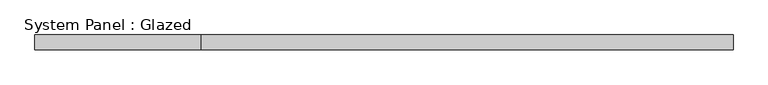
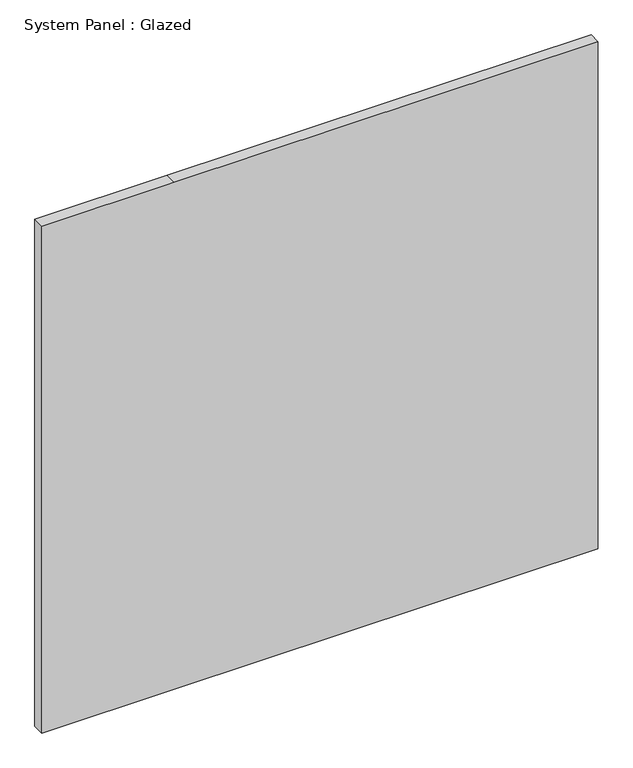
"""IFC4 building model written with IfcOpenShell, lengths in millimetres: plate geometry, System Panel : Glazed."""

from ifc_helpers import new_model, si_unit, frame, origin, place, context, project, spatial, polyline, outline, extrude, source, transform, mapped, element, save


def system_panel_glazed_8fe2fc81(model_context):
    return source(origin(), model_context, "Body", "SweptSolid", [
        extrude(outline(polyline([(0.0, -600.075), (0.0, -314.325), (0.0, 600.075), (1155.7, 600.075), (1155.7, -314.325), (1155.7, -600.075), (0.0, -600.075)])), frame((0.0, -44.45, 0.0), z_axis=(0.0, 1.0, 0.0), x_axis=(0.0, 0.0, 1.0)), (0.0, 0.0, 1.0), 25.4),
    ])


if __name__ == "__main__":
    model = new_model("IFC4")
    model_context = context("Model", 3, world=origin())
    ifc_project = project(units=[si_unit("LENGTHUNIT", "METRE", prefix="MILLI")], contexts=[model_context])
    site = spatial("IfcSite", under=ifc_project)
    building = spatial("IfcBuilding", under=site)
    placement = place(None, origin())
    system_panel_glazed_shape = system_panel_glazed_8fe2fc81(model_context)
    element("IfcPlate", 1, ObjectType="System Panel : Glazed", at=placement, inside=building, context=model_context, shape_type="MappedRepresentation", body=[
        mapped(system_panel_glazed_shape, transform((0.0, 0.0, 0.0), x_axis=(1.0, 0.0, 0.0), y_axis=(0.0, 1.0, 0.0), z_axis=(0.0, 0.0, 1.0))),
    ])
    save(model, "model.ifc")

# Revit data of these elements
# Type "System Panel : Glazed"
#   Construction Type Id = "GSP4R"
#   Analytic Construction = "1/8 in Pilkington single glazing"
#   Visual Light Transmittance = 0.9
#   Solar Heat Gain Coefficient = 0.86
#   Heat Transfer Coefficient (U) = 1.18115 BTU/(h·ft²·°F)
#   Define Thermal Properties by = 1
# Element 1 (IfcPlate, "System Panel : Glazed")
#   Materials on its faces: "Glass"
# Materials
#   "Glass": class "Glass", colour RGB 0 128 192, transparency 0.75, Description = "Soda Lime Glass", Cost = 0
